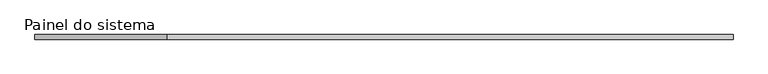
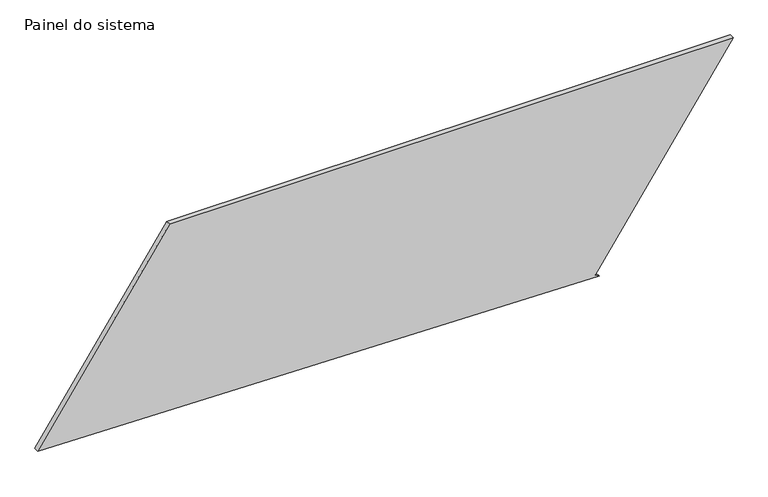
"""IFC4 building model written with IfcOpenShell, lengths in millimetres: plate geometry, Painel do sistema : Envidraçado."""

import ifcopenshell
import ifcopenshell.guid

model = None  # the IFC model being written
_history = None  # IfcOwnerHistory: only IFC2X3 demands one
_inside = {}  # id of a spatial element -> (the spatial element, [elements in it])
_under = {}  # id of a project, library or spatial element -> (it, [spatial elements below it])
_declared = {}  # id of a project -> (the project, [libraries it declares])
_typed = {}  # id of a type object -> (the type object, [elements of that type])
_made_of = {}  # id of a material, layer set ... -> (it, [elements and type objects made of it])


def new_model(schema):
    """Start an empty IFC model of exactly this schema.

    Asked for "IFC4X3", IfcOpenShell would pick the latest addendum, in which some entities
    have other attributes; the version numbers below select the first issue.
    IFC2X3 requires an IfcOwnerHistory on every rooted entity: one is made here for all.
    """
    global model, _history
    if schema == "IFC4X3":
        model = ifcopenshell.file(schema_version=(4, 3, 0, 0))
    else:
        model = ifcopenshell.file(schema=schema)
    _inside.clear()
    _under.clear()
    _declared.clear()
    _typed.clear()
    _made_of.clear()
    _history = None
    if model.schema == "IFC2X3":
        org = make("IfcOrganization", Name="unknown")
        user = make(
            "IfcPersonAndOrganization",
            ThePerson=make("IfcPerson", FamilyName="unknown"),
            TheOrganization=org,
        )
        app = make(
            "IfcApplication",
            ApplicationDeveloper=org,
            Version="unknown",
            ApplicationFullName="unknown",
            ApplicationIdentifier="unknown",
        )
        _history = make(
            "IfcOwnerHistory",
            OwningUser=user,
            OwningApplication=app,
            ChangeAction="ADDED",
            CreationDate=0,
        )
    return model


def make(cls, **values):
    """One entity of the class cls with the attributes given. An attribute that is None is left unset."""
    return model.create_entity(
        cls, **{name: value for name, value in values.items() if value is not None}
    )


def rooted(cls, **values):
    """An entity with a GlobalId (a new one), such as an element, a storey or a relation."""
    return make(cls, GlobalId=ifcopenshell.guid.new(), OwnerHistory=_history, **values)


def si_unit(unit_type, name, prefix=None):
    """IfcSIUnit, for example si_unit("LENGTHUNIT", "METRE", prefix="MILLI")."""
    return make("IfcSIUnit", UnitType=unit_type, Prefix=prefix, Name=name)


def assignment(units):
    """IfcUnitAssignment: the units of a project."""
    return None if units is None else make("IfcUnitAssignment", Units=units)


def point(xyz):
    """IfcCartesianPoint."""
    return None if xyz is None else make("IfcCartesianPoint", Coordinates=xyz)


def direction(xyz):
    """IfcDirection."""
    return None if xyz is None else make("IfcDirection", DirectionRatios=xyz)


def frame(location, z_axis=None, x_axis=None):
    """IfcAxis2Placement3D, a coordinate frame: its origin and axes. An axis left out is left unset."""
    return make(
        "IfcAxis2Placement3D",
        Location=point(location),
        Axis=direction(z_axis),
        RefDirection=direction(x_axis),
    )


def origin():
    """The frame at (0, 0, 0) with its axes left unset."""
    return frame((0.0, 0.0, 0.0))


def place(relative_to, where):
    """IfcLocalPlacement: puts the frame where relative to a parent placement (None: the world)."""
    return make(
        "IfcLocalPlacement", PlacementRelTo=relative_to, RelativePlacement=where
    )


def context(
    kind, dimensions, precision=None, world=None, true_north=None, identifier=None
):
    """IfcGeometricRepresentationContext, for example the 3D "Model" context."""
    return make(
        "IfcGeometricRepresentationContext",
        ContextIdentifier=identifier,
        ContextType=kind,
        CoordinateSpaceDimension=dimensions,
        Precision=precision,
        WorldCoordinateSystem=world,
        TrueNorth=true_north,
    )


def project(units=None, contexts=None):
    """IfcProject with its units and contexts."""
    return rooted(
        "IfcProject",
        Name="project",
        RepresentationContexts=contexts,
        UnitsInContext=assignment(units),
    )


def spatial(cls, under=None, at=None, **own):
    """A site, building, storey or space (cls), placed at a placement, below another one or the project."""
    s = rooted(cls, ObjectPlacement=at, **own)
    if under is not None:
        _under.setdefault(under.id(), (under, []))[1].append(s)
    return s


def polyline(points):
    """IfcPolyline through the points."""
    return make("IfcPolyline", Points=[point(p) for p in points])


def outline(outer, holes=None, kind="AREA"):
    """IfcArbitraryClosedProfileDef: a profile drawn as a closed curve; with holes, ...WithVoids."""
    if holes is None:
        return make("IfcArbitraryClosedProfileDef", ProfileType=kind, OuterCurve=outer)
    return make(
        "IfcArbitraryProfileDefWithVoids",
        ProfileType=kind,
        OuterCurve=outer,
        InnerCurves=holes,
    )


def extrude(swept, where, along, depth):
    """IfcExtrudedAreaSolid: the profile swept, set in the frame where, extruded along a direction by depth."""
    return make(
        "IfcExtrudedAreaSolid",
        SweptArea=swept,
        Position=where,
        ExtrudedDirection=direction(along),
        Depth=depth,
    )


def shape(context_of_items, identifier, shape_type, items):
    """IfcShapeRepresentation: the items that make up one representation, for example the "Body"."""
    return make(
        "IfcShapeRepresentation",
        ContextOfItems=context_of_items,
        RepresentationIdentifier=identifier,
        RepresentationType=shape_type,
        Items=items,
    )


def source(mapping_origin, context_of_items, identifier, shape_type, items):
    """IfcRepresentationMap: a shape defined once, which mapped items show again and again."""
    return make(
        "IfcRepresentationMap",
        MappingOrigin=mapping_origin,
        MappedRepresentation=shape(context_of_items, identifier, shape_type, items),
    )


def transform(
    local_origin,
    x_axis=None,
    y_axis=None,
    z_axis=None,
    scale=None,
    scale2=None,
    scale3=None,
    uniform=True,
):
    """IfcCartesianTransformationOperator3D, or its non-uniform kind. x_axis, y_axis, z_axis: its Axis1, 2, 3."""
    if uniform:
        return make(
            "IfcCartesianTransformationOperator3D",
            Axis1=direction(x_axis),
            Axis2=direction(y_axis),
            LocalOrigin=point(local_origin),
            Scale=scale,
            Axis3=direction(z_axis),
        )
    return make(
        "IfcCartesianTransformationOperator3DnonUniform",
        Axis1=direction(x_axis),
        Axis2=direction(y_axis),
        LocalOrigin=point(local_origin),
        Scale=scale,
        Axis3=direction(z_axis),
        Scale2=scale2,
        Scale3=scale3,
    )


def mapped(mapping_source, mapping_target):
    """IfcMappedItem: shows the shape of a source again, moved by a transform."""
    return make(
        "IfcMappedItem", MappingSource=mapping_source, MappingTarget=mapping_target
    )


def made_of(thing, what):
    """Note that an element or type object is made of a material, layer set ...; save() writes the relation."""
    if what is not None:
        _made_of.setdefault(what.id(), (what, []))[1].append(thing)
    return thing


def element(
    cls,
    number,
    at=None,
    inside=None,
    cuts=None,
    type_object=None,
    material=None,
    context=None,
    identifier="Body",
    shape_type=None,
    held_by="IfcProductDefinitionShape",
    body=None,
    shapes=None,
    **own,
):
    """One element of the class cls, such as IfcWall. Its Tag is "e" and its number.

    at: its placement. inside: the storey or other place that contains it. cuts: it is an
    opening in that element (IfcRelVoidsElement). A single representation is given by context,
    identifier, shape_type and body (its items); several are given by shapes. held_by: the class
    of the entity that holds the representations. save() writes the other relations.
    """
    e = rooted(cls, Tag="e%d" % number, ObjectPlacement=at, **own)
    if body is not None:
        shapes = [shape(context, identifier, shape_type, body)]
    if shapes is not None:
        e.Representation = make(held_by, Representations=shapes)
    if inside is not None:
        _inside.setdefault(inside.id(), (inside, []))[1].append(e)
    if cuts is not None:
        rooted(
            "IfcRelVoidsElement", RelatingBuildingElement=cuts, RelatedOpeningElement=e
        )
    if type_object is not None:
        _typed.setdefault(type_object.id(), (type_object, []))[1].append(e)
    return made_of(e, material)


def aggregate(whole, parts):
    """IfcRelAggregates: a whole, such as a stair, and the parts it consists of."""
    return rooted("IfcRelAggregates", RelatingObject=whole, RelatedObjects=parts)


def save(model, path):
    """Write the relations noted so far, then the file.

    IfcRelAggregates (storeys below a building ...), IfcRelContainedInSpatialStructure (elements
    in a storey), IfcRelDefinesByType, IfcRelAssociatesMaterial and IfcRelDeclares: one each for
    every whole, place, type object, material and project.
    """
    for whole, parts in _under.values():
        aggregate(whole, parts)
    for where, things in _inside.values():
        rooted(
            "IfcRelContainedInSpatialStructure",
            RelatedElements=things,
            RelatingStructure=where,
        )
    for kind, things in _typed.values():
        rooted("IfcRelDefinesByType", RelatedObjects=things, RelatingType=kind)
    for what, things in _made_of.values():
        rooted("IfcRelAssociatesMaterial", RelatedObjects=things, RelatingMaterial=what)
    for by, libraries in _declared.values():
        rooted("IfcRelDeclares", RelatingContext=by, RelatedDefinitions=libraries)
    model.write(path)


def painel_do_sistema_b94b22be(model_context):
    return source(origin(), model_context, "Body", "SweptSolid", [
        extrude(outline(polyline([(0.0, 1167.9283611), (14.052453, 1147.2515972), (1122.8505123, 1900.8188702), (1122.8505123, -1179.4853851), (61.4812132, -1900.8188702), (0.0, 1167.9283611)])), frame((0.0, 24.5, 0.0), z_axis=(0.0, 1.0, 0.0), x_axis=(0.0, 0.0, 1.0)), (0.0, 0.0, 1.0), 25.0),
    ])


if __name__ == "__main__":
    model = new_model("IFC4")
    model_context = context("Model", 3, world=origin())
    ifc_project = project(units=[si_unit("LENGTHUNIT", "METRE", prefix="MILLI")], contexts=[model_context])
    site = spatial("IfcSite", under=ifc_project)
    building = spatial("IfcBuilding", under=site)
    placement = place(None, origin())
    painel_do_sistema_shape = painel_do_sistema_b94b22be(model_context)
    element("IfcPlate", 1, ObjectType="Painel do sistema : Envidraçado", at=placement, inside=building, context=model_context, shape_type="MappedRepresentation", body=[
        mapped(painel_do_sistema_shape, transform((0.0, 0.0, 0.0), x_axis=(1.0, 0.0, 0.0), y_axis=(0.0, 1.0, 0.0), z_axis=(0.0, 0.0, 1.0))),
    ])
    save(model, "model.ifc")

# Revit data of these elements
# Type "Painel do sistema : Envidraçado"
#   Construction Type Id = "GSP4R"
#   Analytic Construction = "Vidraça única Pilkington 1/8 pol"
#   Visual Light Transmittance = 0.9
#   Solar Heat Gain Coefficient = 0.86
#   Heat Transfer Coefficient (U) = 6.7069 W/(m²·K)
# Element 1 (IfcPlate, "Painel do sistema : Envidraçado")
#   Materials on its faces: "Vidro"
# Materials
#   "Vidro": class "Vidro", colour RGB 0 128 192, transparency 0.9, Description = "Vidro de sílica", Cost = 0
